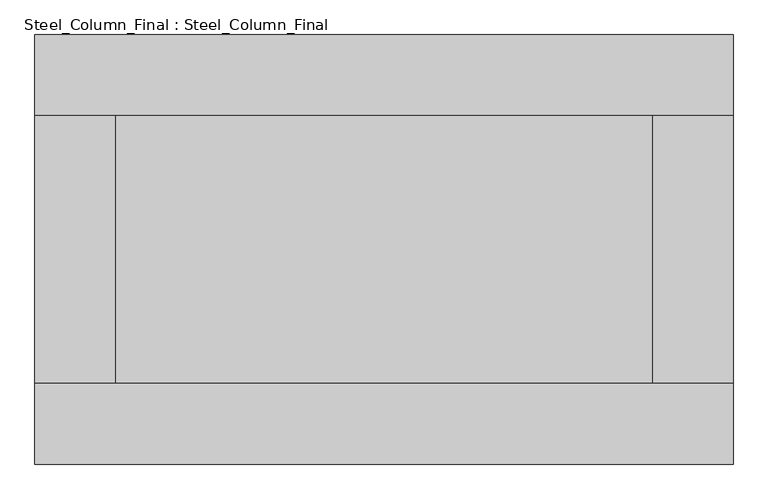
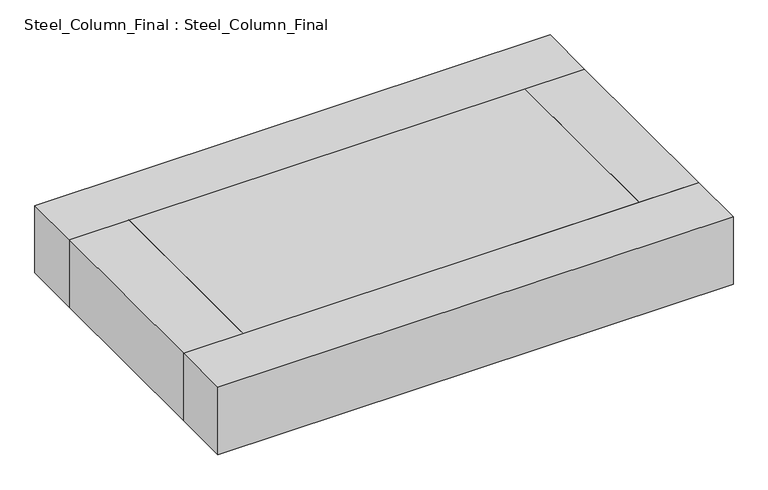
"""IFC4 building model written with IfcOpenShell, lengths in millimetres: proxy geometry, Steel_Column_Final : Steel_Column_Final."""

from ifc_helpers import new_model, si_unit, frame, origin, place, context, project, spatial, polyline, outline, extrude, source, transform, mapped, element, save


def steel_column_final_steel_column_final_9c8beafe(model_context):
    return source(origin(), model_context, "Body", "SweptSolid", [
        extrude(outline(polyline([(6500.0, 2500.0), (-6500.0, 2500.0), (-6500.0, 4000.0), (6500.0, 4000.0), (6500.0, 2500.0)])), frame((0.0, 0.0, 9590.0), z_axis=(0.0, 0.0, 1.0), x_axis=(1.0, 0.0, 0.0)), (0.0, 0.0, 1.0), 1800.0),
        extrude(outline(polyline([(-6500.0, -2500.0), (6500.0, -2500.0), (6500.0, -4000.0), (-6500.0, -4000.0), (-6500.0, -2500.0)])), frame((0.0, 0.0, 9590.0), z_axis=(0.0, 0.0, 1.0), x_axis=(1.0, 0.0, 0.0)), (0.0, 0.0, 1.0), 1800.0),
        extrude(outline(polyline([(5000.0, -2500.0), (5000.0, 2500.0), (6500.0, 2500.0), (6500.0, -2500.0), (5000.0, -2500.0)])), frame((0.0, 0.0, 9590.0), z_axis=(0.0, 0.0, 1.0), x_axis=(1.0, 0.0, 0.0)), (0.0, 0.0, 1.0), 1800.0),
        extrude(outline(polyline([(-5000.0, 2500.0), (-5000.0, -2500.0), (-6500.0, -2500.0), (-6500.0, 2500.0), (-5000.0, 2500.0)])), frame((0.0, 0.0, 9590.0), z_axis=(0.0, 0.0, 1.0), x_axis=(1.0, 0.0, 0.0)), (0.0, 0.0, 1.0), 1800.0),
        extrude(outline(polyline([(-5000.0, -2500.0), (-5000.0, 2500.0), (5000.0, 2500.0), (5000.0, -2500.0), (-5000.0, -2500.0)])), frame((0.0, 0.0, 9590.0), z_axis=(0.0, 0.0, 1.0), x_axis=(1.0, 0.0, 0.0)), (0.0, 0.0, 1.0), 1800.0),
    ])


if __name__ == "__main__":
    model = new_model("IFC4")
    model_context = context("Model", 3, world=origin())
    ifc_project = project(units=[si_unit("LENGTHUNIT", "METRE", prefix="MILLI")], contexts=[model_context])
    site = spatial("IfcSite", under=ifc_project)
    building = spatial("IfcBuilding", under=site)
    placement = place(None, origin())
    steel_column_final_steel_column_final_shape = steel_column_final_steel_column_final_9c8beafe(model_context)
    element("IfcBuildingElementProxy", 1, Name="Steel_Column_Final : Steel_Column_Final", ObjectType="Steel_Column_Final : Steel_Column_Final", at=placement, inside=building, context=model_context, shape_type="MappedRepresentation", body=[
        mapped(steel_column_final_steel_column_final_shape, transform((0.0, 0.0, 0.0), x_axis=(1.0, 0.0, 0.0), y_axis=(0.0, 1.0, 0.0), z_axis=(0.0, 0.0, 1.0))),
    ])
    save(model, "model.ifc")

# Revit data of these elements
# Type "Steel_Column_Final : Steel_Column_Final"
#   Top Width [instance default] = 5000 mm
#   Top Length = 10000 mm
#   Length = 21000 mm
#   Height [instance default] = 50000 mm
#   Bottom Width [instance default] = 5000 mm
#   Default Elevation = 0
# Element 1 (IfcBuildingElementProxy, "Steel_Column_Final : Steel_Column_Final")
#   Height = 9590 mm
